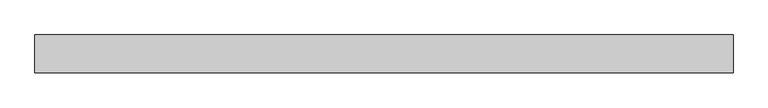
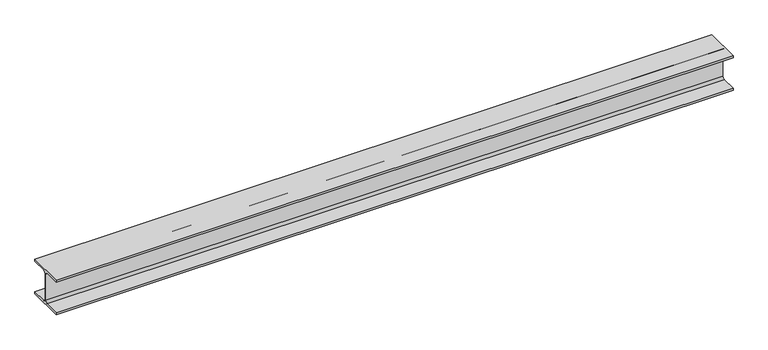
"""IFC4 building model written with IfcOpenShell, lengths in millimetres: beam geometry, 0912_Steel Framing_H-KSD3502 : H_SB_ASB_H-200x200x8x12."""

from ifc_helpers import new_model, si_unit, point, frame, frame_2d, origin, place, context, project, spatial, polyline, circle_curve, trimmed, segment, composite_curve, outline, extrude, source, transform, mapped, element, save


def beam_cdd6222a(model_context):
    return source(origin(), model_context, "Body", "SweptSolid", [
        extrude(outline(composite_curve([segment(polyline([(-100.0, -88.0), (-17.0, -88.0)]), True, "CONTINUOUS"), segment(trimmed(circle_curve(frame_2d((-17.0, -75.0)), 13.0), [point((-17.0, -88.0))], [point((-4.0, -75.0))], True, "CARTESIAN"), True, "CONTINUOUS"), segment(polyline([(-4.0, -75.0), (-4.0, 75.0)]), True, "CONTINUOUS"), segment(trimmed(circle_curve(frame_2d((-17.0, 75.0)), 13.0), [point((-4.0, 75.0))], [point((-17.0, 88.0))], True, "CARTESIAN"), True, "CONTINUOUS"), segment(polyline([(-17.0, 88.0), (-100.0, 88.0), (-100.0, 100.0), (100.0, 100.0), (100.0, 88.0), (17.0, 88.0)]), True, "CONTINUOUS"), segment(trimmed(circle_curve(frame_2d((17.0, 75.0)), 13.0), [point((17.0, 88.0))], [point((4.0, 75.0))], True, "CARTESIAN"), True, "CONTINUOUS"), segment(polyline([(4.0, 75.0), (4.0, -75.0)]), True, "CONTINUOUS"), segment(trimmed(circle_curve(frame_2d((17.0, -75.0)), 13.0), [point((4.0, -75.0))], [point((17.0, -88.0))], True, "CARTESIAN"), True, "CONTINUOUS"), segment(polyline([(17.0, -88.0), (100.0, -88.0), (100.0, -100.0), (-100.0, -100.0), (-100.0, -88.0)]), True, "CONTINUOUS")], self_intersect=False)), frame((-1862.5629181, 0.0, 0.0), z_axis=(1.0, 0.0, 0.0), x_axis=(0.0, 1.0, 0.0)), (0.0, 0.0, 1.0), 3701.2673573),
    ])


if __name__ == "__main__":
    model = new_model("IFC4")
    model_context = context("Model", 3, world=origin())
    ifc_project = project(units=[si_unit("LENGTHUNIT", "METRE", prefix="MILLI")], contexts=[model_context])
    site = spatial("IfcSite", under=ifc_project)
    building = spatial("IfcBuilding", under=site)
    placement = place(None, origin())
    beam_shape = beam_cdd6222a(model_context)
    element("IfcBeam", 1, ObjectType="0912_Steel Framing_H-KSD3502 : H_SB_ASB_H-200x200x8x12", at=placement, inside=building, context=model_context, shape_type="MappedRepresentation", body=[
        mapped(beam_shape, transform((0.0, 0.0, 0.0), x_axis=(1.0, 0.0, 0.0), y_axis=(0.0, 1.0, 0.0), z_axis=(0.0, 0.0, 1.0))),
    ])
    save(model, "model.ifc")

# Revit data of these elements
# Type "0912_Steel Framing_H-KSD3502 : H_SB_ASB_H-200x200x8x12"
#   H_WM Code_1 = "S01AA002-00001 | Main Steel Structure Fabrication Work | Shelter/Building | Medium Steel - Standard (90KG/M>Weight≥30KG/M) | Material: (   )"
#   H_WM Code_2 = "S03AA028-00001 | Main Steel Structure Erection Work | Shelter/Building | Medium Steel (90KG/M>Weight≥30KG/M) | Material: (   )"
#   H_WM Code_3 = "S01AA010-00001 | Main Steel Structure Fabrication Work | Shelter/Building | Steel Painting/Coating | for Non-Fireproofed Steel Surface, Surface Preparation, Primer, Second & Final Coat | Material: (   )"
#   H_Q'ty Cal Type Tag = "SB-Q2"
#   Width = 20.0 cm
#   Web Thickness = 0.8 cm
#   Web Fillet = 1.3 cm
#   Warping Constant = 141000.0 cm⁶
#   W = 0
#   Torsional Moment of Inertia = 26.2485 cm⁴
#   Section Area = 63.53 cm²
#   Plastic Modulus weak axis = 244.0 cm³
#   Plastic Modulus strong axis = 525.0 cm³
#   Perimeter = 1.16 m²/m
#   Nominal Weight = 49.90 kgf/m
#   Moment of Inertia weak axis = 1600.00 cm⁴
#   Moment of Inertia strong axis = 4720.00 cm⁴
#   Height = 20.0 cm
#   Flange Thickness = 1.2 cm
#   Elastic Modulus weak axis = 160.0 cm³
#   Elastic Modulus strong axis = 472.0 cm³
#   Centroid Vertical = 10.0 cm
#   Centroid Horizontal = 10.0 cm
#   Ix = 47200000
#   Length [instance default] = 1.5240 m
#   Zx = 525000
#   b = 0.2000 m
#   h = 0.2000 m
#   r = 0.0130 m
#   s = 0.0080 m
#   t = 0.0120 m
#   A = 0.006353 m²
#   Structural Material [instance default] = Steel, 45-345
#   Assembly Code = ""
# Element 1 (IfcBeam, "0912_Steel Framing_H-KSD3502 : H_SB_ASB_H-200x200x8x12")
#   Structural Material = none
# Materials
#   "Steel, 45-345": class "Metal", colour RGB 189 187 185, transparency 0, Description = "Steel 345 MPa", Cost = 0
